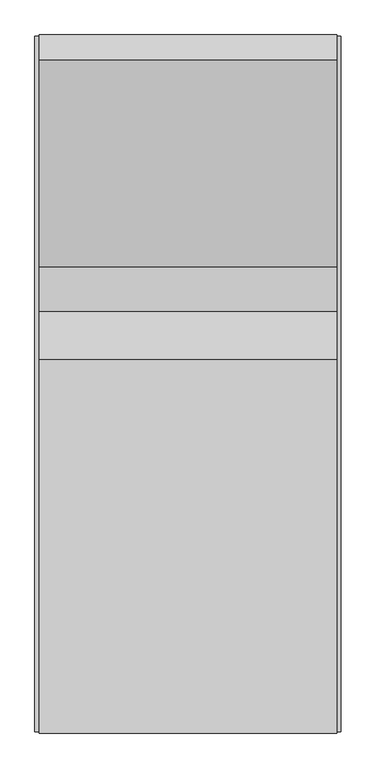
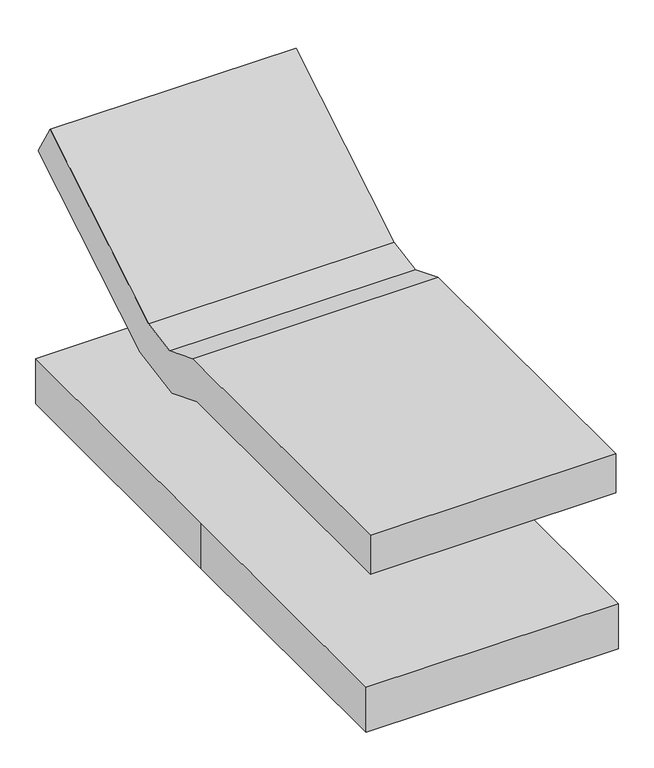
"""IFC4 building model written with IfcOpenShell, lengths in millimetres: proxy geometry, M3025 - Mattress, Pressure Reduction : M3025 - Mattress, Pressure Reduction."""

from ifc_helpers import new_model, si_unit, frame, origin, origin_with_axes, place, context, project, spatial, polyline, outline, extrude, source, transform, mapped, element, save


def specialty_equipment_fde20e22(model_context):
    return source(origin(), model_context, "Body", "SweptSolid", [
        extrude(outline(polyline([(46.7880485, 621.3510043), (-1070.8119515, 621.3510043), (-1070.8119515, 773.7510043), (76.013804, 773.7510043), (222.4258933, 715.4521116), (359.5657775, 739.6335733), (992.3201489, 1119.8307566), (1070.8119515, 989.19846), (413.846315, 594.4536809), (206.2622208, 557.8510043), (46.7880485, 621.3510043)])), frame((-457.2, 0.0, 0.0), z_axis=(1.0, 0.0, 0.0), x_axis=(0.0, 1.0, 0.0)), (0.0, 0.0, 1.0), 914.4),
        extrude(outline(polyline([(-469.9, 1066.8), (469.9, 1066.8), (469.9, -1066.8), (-469.9, -1066.8), (-469.9, 0.0), (-469.9, 1066.8)])), origin_with_axes(), (0.0, 0.0, 1.0), 177.8),
    ])


if __name__ == "__main__":
    model = new_model("IFC4")
    model_context = context("Model", 3, world=origin())
    ifc_project = project(units=[si_unit("LENGTHUNIT", "METRE", prefix="MILLI")], contexts=[model_context])
    site = spatial("IfcSite", under=ifc_project)
    building = spatial("IfcBuilding", under=site)
    placement = place(None, origin())
    specialty_equipment_shape = specialty_equipment_fde20e22(model_context)
    element("IfcBuildingElementProxy", 1, Name="M3025 - Mattress, Pressure Reduction : M3025 - Mattress, Pressure Reduction", ObjectType="M3025 - Mattress, Pressure Reduction : M3025 - Mattress, Pressure Reduction", at=placement, inside=building, context=model_context, shape_type="MappedRepresentation", body=[
        mapped(specialty_equipment_shape, transform((0.0, 0.0, 0.0), x_axis=(1.0, 0.0, 0.0), y_axis=(0.0, 1.0, 0.0), z_axis=(0.0, 0.0, 1.0))),
    ])
    save(model, "model.ifc")

# Revit data of these elements
# Type "M3025 - Mattress, Pressure Reduction : M3025 - Mattress, Pressure Reduction"
#   Watts2 = "0"
#   Watts1 = "0"
#   Unit_Issue = "EA"
#   UTIL_6_Misc = "-"
#   UTIL_5_NonMedGas = "-"
#   UTIL_4_MiscGas = "-"
#   UTIL_3_MedGas = "-"
#   UTIL_2_Elec = "A"
#   UTIL_1_WaterDrain = "-"
#   Nomenclature = "Mattress, Pressure Reduction"
#   NSN = "6530"
#   Location [instance default] = ""
#   JSN = "M3025"
#   Fund_Source_VA = "-"
#   Fund_Source_Navy = "-"
#   Fund_Source_Army = "-"
#   Fund_Source_AF = "-"
#   ELEC_Volts2 = "0"
#   ELEC_Volts1 = "0"
#   ELEC_Phase2 = "0"
#   ELEC_Phase1 = "0"
#   ELEC_HertzSwitch = "0"
#   ELEC_HertzDependent = "0"
#   ELEC_Hertz = "0"
#   ELEC_Amps2 = "0"
#   ELEC_Amps1 = "0"
#   DetailDescription = "Pressure reduction mattress. Consists of polyurethane foam and air or gel cylinders to spread pressure of patient's body weight across a larger surface area. Some models have electric pumps for inflation and pressure adjustment; other manufacturers score the foam to distribute pressure. Used to prevent bed sores from developing and promote the healing of ulcers. Unit also relieves patient stress by reducing the amount of required patient turning. All-gel and all-foam mattresses as well as comparably therapeutic low air loss mattress systems are available."
#   CAT_VA = "C"
#   CAT_Navy = "C"
#   CAT_IHS = "-"
#   CAT_Army = "C"
#   CAT_AF = "C"
#   BTUperhour = "0"
#   Weight_IP = 47
#   DIM_Width_IP = 3' - 1"
#   DIM_Height_IP = 0' - 7"
#   DIM_Depth_IP = 7' - 0"
# Element 1 (IfcBuildingElementProxy, "M3025 - Mattress, Pressure Reduction : M3025 - Mattress, Pressure Reduction")
#   Materials on its faces: "EquipSpace"
# Materials
#   "EquipSpace": class "Unassigned", colour RGB 221 217 195, transparency 0.5
